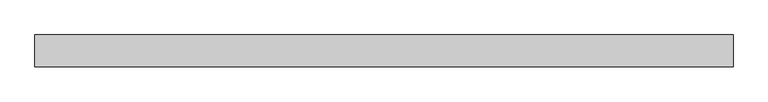
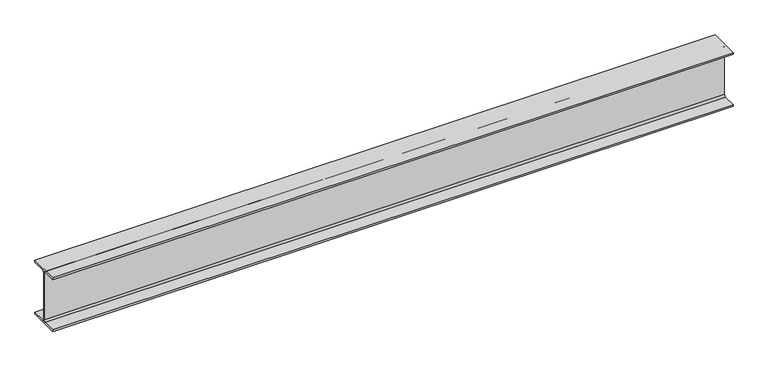
"""IFC4 building model written with IfcOpenShell, lengths in millimetres: beam geometry, Steel Beam_H-KSD3502 : H_SB_ASB_H-200x200x8x12."""

import ifcopenshell
import ifcopenshell.guid

model = None  # the IFC model being written
_history = None  # IfcOwnerHistory: only IFC2X3 demands one
_inside = {}  # id of a spatial element -> (the spatial element, [elements in it])
_under = {}  # id of a project, library or spatial element -> (it, [spatial elements below it])
_declared = {}  # id of a project -> (the project, [libraries it declares])
_typed = {}  # id of a type object -> (the type object, [elements of that type])
_made_of = {}  # id of a material, layer set ... -> (it, [elements and type objects made of it])


def new_model(schema):
    """Start an empty IFC model of exactly this schema.

    Asked for "IFC4X3", IfcOpenShell would pick the latest addendum, in which some entities
    have other attributes; the version numbers below select the first issue.
    IFC2X3 requires an IfcOwnerHistory on every rooted entity: one is made here for all.
    """
    global model, _history
    if schema == "IFC4X3":
        model = ifcopenshell.file(schema_version=(4, 3, 0, 0))
    else:
        model = ifcopenshell.file(schema=schema)
    _inside.clear()
    _under.clear()
    _declared.clear()
    _typed.clear()
    _made_of.clear()
    _history = None
    if model.schema == "IFC2X3":
        org = make("IfcOrganization", Name="unknown")
        user = make(
            "IfcPersonAndOrganization",
            ThePerson=make("IfcPerson", FamilyName="unknown"),
            TheOrganization=org,
        )
        app = make(
            "IfcApplication",
            ApplicationDeveloper=org,
            Version="unknown",
            ApplicationFullName="unknown",
            ApplicationIdentifier="unknown",
        )
        _history = make(
            "IfcOwnerHistory",
            OwningUser=user,
            OwningApplication=app,
            ChangeAction="ADDED",
            CreationDate=0,
        )
    return model


def make(cls, **values):
    """One entity of the class cls with the attributes given. An attribute that is None is left unset."""
    return model.create_entity(
        cls, **{name: value for name, value in values.items() if value is not None}
    )


def rooted(cls, **values):
    """An entity with a GlobalId (a new one), such as an element, a storey or a relation."""
    return make(cls, GlobalId=ifcopenshell.guid.new(), OwnerHistory=_history, **values)


def si_unit(unit_type, name, prefix=None):
    """IfcSIUnit, for example si_unit("LENGTHUNIT", "METRE", prefix="MILLI")."""
    return make("IfcSIUnit", UnitType=unit_type, Prefix=prefix, Name=name)


def assignment(units):
    """IfcUnitAssignment: the units of a project."""
    return None if units is None else make("IfcUnitAssignment", Units=units)


def point(xyz):
    """IfcCartesianPoint."""
    return None if xyz is None else make("IfcCartesianPoint", Coordinates=xyz)


def direction(xyz):
    """IfcDirection."""
    return None if xyz is None else make("IfcDirection", DirectionRatios=xyz)


def frame(location, z_axis=None, x_axis=None):
    """IfcAxis2Placement3D, a coordinate frame: its origin and axes. An axis left out is left unset."""
    return make(
        "IfcAxis2Placement3D",
        Location=point(location),
        Axis=direction(z_axis),
        RefDirection=direction(x_axis),
    )


def frame_2d(location, x_axis=None):
    """IfcAxis2Placement2D, a coordinate frame in the plane: its origin and x axis."""
    return make(
        "IfcAxis2Placement2D", Location=point(location), RefDirection=direction(x_axis)
    )


def origin():
    """The frame at (0, 0, 0) with its axes left unset."""
    return frame((0.0, 0.0, 0.0))


def place(relative_to, where):
    """IfcLocalPlacement: puts the frame where relative to a parent placement (None: the world)."""
    return make(
        "IfcLocalPlacement", PlacementRelTo=relative_to, RelativePlacement=where
    )


def context(
    kind, dimensions, precision=None, world=None, true_north=None, identifier=None
):
    """IfcGeometricRepresentationContext, for example the 3D "Model" context."""
    return make(
        "IfcGeometricRepresentationContext",
        ContextIdentifier=identifier,
        ContextType=kind,
        CoordinateSpaceDimension=dimensions,
        Precision=precision,
        WorldCoordinateSystem=world,
        TrueNorth=true_north,
    )


def project(units=None, contexts=None):
    """IfcProject with its units and contexts."""
    return rooted(
        "IfcProject",
        Name="project",
        RepresentationContexts=contexts,
        UnitsInContext=assignment(units),
    )


def spatial(cls, under=None, at=None, **own):
    """A site, building, storey or space (cls), placed at a placement, below another one or the project."""
    s = rooted(cls, ObjectPlacement=at, **own)
    if under is not None:
        _under.setdefault(under.id(), (under, []))[1].append(s)
    return s


def polyline(points):
    """IfcPolyline through the points."""
    return make("IfcPolyline", Points=[point(p) for p in points])


def circle_curve(where, radius):
    """IfcCircle in the frame where."""
    return make("IfcCircle", Position=where, Radius=radius)


def trimmed(basis, trim1, trim2, sense, master):
    """IfcTrimmedCurve: the piece of a basis curve between two trims."""
    return make(
        "IfcTrimmedCurve",
        BasisCurve=basis,
        Trim1=trim1,
        Trim2=trim2,
        SenseAgreement=sense,
        MasterRepresentation=master,
    )


def segment(curve, same_sense, transition):
    """IfcCompositeCurveSegment."""
    return make(
        "IfcCompositeCurveSegment",
        Transition=transition,
        SameSense=same_sense,
        ParentCurve=curve,
    )


def composite_curve(segments, self_intersect=None):
    """IfcCompositeCurve: segments joined end to end."""
    return make("IfcCompositeCurve", Segments=segments, SelfIntersect=self_intersect)


def outline(outer, holes=None, kind="AREA"):
    """IfcArbitraryClosedProfileDef: a profile drawn as a closed curve; with holes, ...WithVoids."""
    if holes is None:
        return make("IfcArbitraryClosedProfileDef", ProfileType=kind, OuterCurve=outer)
    return make(
        "IfcArbitraryProfileDefWithVoids",
        ProfileType=kind,
        OuterCurve=outer,
        InnerCurves=holes,
    )


def extrude(swept, where, along, depth):
    """IfcExtrudedAreaSolid: the profile swept, set in the frame where, extruded along a direction by depth."""
    return make(
        "IfcExtrudedAreaSolid",
        SweptArea=swept,
        Position=where,
        ExtrudedDirection=direction(along),
        Depth=depth,
    )


def shape(context_of_items, identifier, shape_type, items):
    """IfcShapeRepresentation: the items that make up one representation, for example the "Body"."""
    return make(
        "IfcShapeRepresentation",
        ContextOfItems=context_of_items,
        RepresentationIdentifier=identifier,
        RepresentationType=shape_type,
        Items=items,
    )


def source(mapping_origin, context_of_items, identifier, shape_type, items):
    """IfcRepresentationMap: a shape defined once, which mapped items show again and again."""
    return make(
        "IfcRepresentationMap",
        MappingOrigin=mapping_origin,
        MappedRepresentation=shape(context_of_items, identifier, shape_type, items),
    )


def transform(
    local_origin,
    x_axis=None,
    y_axis=None,
    z_axis=None,
    scale=None,
    scale2=None,
    scale3=None,
    uniform=True,
):
    """IfcCartesianTransformationOperator3D, or its non-uniform kind. x_axis, y_axis, z_axis: its Axis1, 2, 3."""
    if uniform:
        return make(
            "IfcCartesianTransformationOperator3D",
            Axis1=direction(x_axis),
            Axis2=direction(y_axis),
            LocalOrigin=point(local_origin),
            Scale=scale,
            Axis3=direction(z_axis),
        )
    return make(
        "IfcCartesianTransformationOperator3DnonUniform",
        Axis1=direction(x_axis),
        Axis2=direction(y_axis),
        LocalOrigin=point(local_origin),
        Scale=scale,
        Axis3=direction(z_axis),
        Scale2=scale2,
        Scale3=scale3,
    )


def mapped(mapping_source, mapping_target):
    """IfcMappedItem: shows the shape of a source again, moved by a transform."""
    return make(
        "IfcMappedItem", MappingSource=mapping_source, MappingTarget=mapping_target
    )


def made_of(thing, what):
    """Note that an element or type object is made of a material, layer set ...; save() writes the relation."""
    if what is not None:
        _made_of.setdefault(what.id(), (what, []))[1].append(thing)
    return thing


def element(
    cls,
    number,
    at=None,
    inside=None,
    cuts=None,
    type_object=None,
    material=None,
    context=None,
    identifier="Body",
    shape_type=None,
    held_by="IfcProductDefinitionShape",
    body=None,
    shapes=None,
    **own,
):
    """One element of the class cls, such as IfcWall. Its Tag is "e" and its number.

    at: its placement. inside: the storey or other place that contains it. cuts: it is an
    opening in that element (IfcRelVoidsElement). A single representation is given by context,
    identifier, shape_type and body (its items); several are given by shapes. held_by: the class
    of the entity that holds the representations. save() writes the other relations.
    """
    e = rooted(cls, Tag="e%d" % number, ObjectPlacement=at, **own)
    if body is not None:
        shapes = [shape(context, identifier, shape_type, body)]
    if shapes is not None:
        e.Representation = make(held_by, Representations=shapes)
    if inside is not None:
        _inside.setdefault(inside.id(), (inside, []))[1].append(e)
    if cuts is not None:
        rooted(
            "IfcRelVoidsElement", RelatingBuildingElement=cuts, RelatedOpeningElement=e
        )
    if type_object is not None:
        _typed.setdefault(type_object.id(), (type_object, []))[1].append(e)
    return made_of(e, material)


def aggregate(whole, parts):
    """IfcRelAggregates: a whole, such as a stair, and the parts it consists of."""
    return rooted("IfcRelAggregates", RelatingObject=whole, RelatedObjects=parts)


def save(model, path):
    """Write the relations noted so far, then the file.

    IfcRelAggregates (storeys below a building ...), IfcRelContainedInSpatialStructure (elements
    in a storey), IfcRelDefinesByType, IfcRelAssociatesMaterial and IfcRelDeclares: one each for
    every whole, place, type object, material and project.
    """
    for whole, parts in _under.values():
        aggregate(whole, parts)
    for where, things in _inside.values():
        rooted(
            "IfcRelContainedInSpatialStructure",
            RelatedElements=things,
            RelatingStructure=where,
        )
    for kind, things in _typed.values():
        rooted("IfcRelDefinesByType", RelatedObjects=things, RelatingType=kind)
    for what, things in _made_of.values():
        rooted("IfcRelAssociatesMaterial", RelatedObjects=things, RelatingMaterial=what)
    for by, libraries in _declared.values():
        rooted("IfcRelDeclares", RelatingContext=by, RelatedDefinitions=libraries)
    model.write(path)


def beam_d849abf2(model_context):
    return source(origin(), model_context, "Body", "SweptSolid", [
        extrude(outline(composite_curve([segment(polyline([(82.5, -141.5), (82.5, -151.7), (-82.5, -151.7), (-82.5, -141.5), (-11.9, -141.5)]), True, "CONTINUOUS"), segment(trimmed(circle_curve(frame_2d((-11.9, -132.6)), 8.9), [point((-11.9, -141.5))], [point((-3.0, -132.6))], True, "CARTESIAN"), True, "CONTINUOUS"), segment(polyline([(-3.0, -132.6), (-3.0, 132.6)]), True, "CONTINUOUS"), segment(trimmed(circle_curve(frame_2d((-11.9, 132.6)), 8.9), [point((-3.0, 132.6))], [point((-11.9, 141.5))], True, "CARTESIAN"), True, "CONTINUOUS"), segment(polyline([(-11.9, 141.5), (-82.5, 141.5), (-82.5, 151.7), (82.5, 151.7), (82.5, 141.5), (11.9, 141.5)]), True, "CONTINUOUS"), segment(trimmed(circle_curve(frame_2d((11.9, 132.6)), 8.9), [point((11.9, 141.5))], [point((3.0, 132.6))], True, "CARTESIAN"), True, "CONTINUOUS"), segment(polyline([(3.0, 132.6), (3.0, -132.6)]), True, "CONTINUOUS"), segment(trimmed(circle_curve(frame_2d((11.9, -132.6)), 8.9), [point((3.0, -132.6))], [point((11.9, -141.5))], True, "CARTESIAN"), True, "CONTINUOUS"), segment(polyline([(11.9, -141.5), (82.5, -141.5)]), True, "CONTINUOUS")], self_intersect=False)), frame((-1850.8543264, 0.0, 0.0), z_axis=(1.0, 0.0, 0.0), x_axis=(0.0, 1.0, 0.0)), (0.0, 0.0, 1.0), 3630.9979746),
    ])


if __name__ == "__main__":
    model = new_model("IFC4")
    model_context = context("Model", 3, world=origin())
    ifc_project = project(units=[si_unit("LENGTHUNIT", "METRE", prefix="MILLI")], contexts=[model_context])
    site = spatial("IfcSite", under=ifc_project)
    building = spatial("IfcBuilding", under=site)
    placement = place(None, origin())
    beam_shape = beam_d849abf2(model_context)
    element("IfcBeam", 1, ObjectType="Steel Beam_H-KSD3502 : H_SB_ASB_H-200x200x8x12", at=placement, inside=building, context=model_context, shape_type="MappedRepresentation", body=[
        mapped(beam_shape, transform((0.0, 0.0, 0.0), x_axis=(1.0, 0.0, 0.0), y_axis=(0.0, 1.0, 0.0), z_axis=(0.0, 0.0, 1.0))),
    ])
    save(model, "model.ifc")

# Revit data of these elements
# Type "Steel Beam_H-KSD3502 : H_SB_ASB_H-200x200x8x12"
#   Width = 20.0 cm
#   Web Thickness = 0.8 cm
#   Web Fillet = 1.3 cm
#   Warping Constant = 141376.0 cm⁶
#   Torsional Moment of Inertia = 26.2485 cm⁴
#   Torsional Modulus = 1.0 cm³
#   Section Area = 63.53 cm²
#   Plastic Modulus weak axis = 244.0 cm³
#   Plastic Modulus strong axis = 525.0 cm³
#   Perimeter = 1.16 m²/m
#   Nominal Weight = 49.90 kgf/m
#   Moment of Inertia weak axis = 1600.00 cm⁴
#   Moment of Inertia strong axis = 4720.00 cm⁴
#   Height = 20.0 cm
#   Flange Thickness = 1.2 cm
#   Elastic Modulus weak axis = 160.0 cm³
#   Elastic Modulus strong axis = 472.0 cm³
#   Centroid Vertical = 10.0 cm
#   Centroid Horizontal = 10.0 cm
#   Length [instance default] = 1.5240 m
#   Structural Material [instance default] = Steel, 45-345
#   Assembly Code = ""
# Element 1 (IfcBeam, "Steel Beam_H-KSD3502 : H_SB_ASB_H-200x200x8x12")
#   Structural Material = none
# Materials
#   "Steel, 45-345": class "Metal", colour RGB 189 187 185, transparency 0, Description = "Steel 345 MPa", Cost = 0
